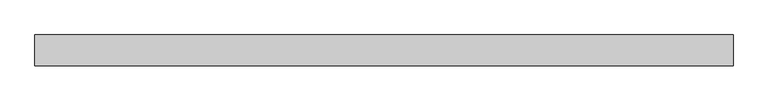
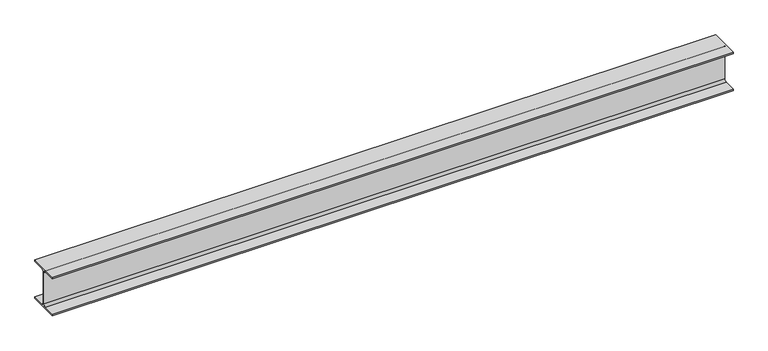
"""IFC4 building model written with IfcOpenShell, lengths in millimetres: beam geometry, 0912_Steel Framing_H-KSD3502 : H_SB_ASB_H-340x250x9x14."""

from ifc_helpers import new_model, si_unit, point, frame, frame_2d, origin, place, context, project, spatial, polyline, circle_curve, trimmed, segment, composite_curve, outline, extrude, source, transform, mapped, element, save


def beam_b7f7b6e9(model_context):
    return source(origin(), model_context, "Body", "SweptSolid", [
        extrude(outline(composite_curve([segment(polyline([(125.0, -156.0), (125.0, -170.0), (-125.0, -170.0), (-125.0, -156.0), (-24.5, -156.0)]), True, "CONTINUOUS"), segment(trimmed(circle_curve(frame_2d((-24.5, -136.0)), 20.0), [point((-24.5, -156.0))], [point((-4.5, -136.0))], True, "CARTESIAN"), True, "CONTINUOUS"), segment(polyline([(-4.5, -136.0), (-4.5, 136.0)]), True, "CONTINUOUS"), segment(trimmed(circle_curve(frame_2d((-24.5, 136.0)), 20.0), [point((-4.5, 136.0))], [point((-24.5, 156.0))], True, "CARTESIAN"), True, "CONTINUOUS"), segment(polyline([(-24.5, 156.0), (-125.0, 156.0), (-125.0, 170.0), (125.0, 170.0), (125.0, 156.0), (24.5, 156.0)]), True, "CONTINUOUS"), segment(trimmed(circle_curve(frame_2d((24.5, 136.0)), 20.0), [point((24.5, 156.0))], [point((4.5, 136.0))], True, "CARTESIAN"), True, "CONTINUOUS"), segment(polyline([(4.5, 136.0), (4.5, -136.0)]), True, "CONTINUOUS"), segment(trimmed(circle_curve(frame_2d((24.5, -136.0)), 20.0), [point((4.5, -136.0))], [point((24.5, -156.0))], True, "CARTESIAN"), True, "CONTINUOUS"), segment(polyline([(24.5, -156.0), (125.0, -156.0)]), True, "CONTINUOUS")], self_intersect=False)), frame((-2837.3, 0.0, 0.0), z_axis=(1.0, 0.0, 0.0), x_axis=(0.0, 1.0, 0.0)), (0.0, 0.0, 1.0), 5674.6),
    ])


if __name__ == "__main__":
    model = new_model("IFC4")
    model_context = context("Model", 3, world=origin())
    ifc_project = project(units=[si_unit("LENGTHUNIT", "METRE", prefix="MILLI")], contexts=[model_context])
    site = spatial("IfcSite", under=ifc_project)
    building = spatial("IfcBuilding", under=site)
    placement = place(None, origin())
    beam_shape = beam_b7f7b6e9(model_context)
    element("IfcBeam", 1, ObjectType="0912_Steel Framing_H-KSD3502 : H_SB_ASB_H-340x250x9x14", at=placement, inside=building, context=model_context, shape_type="MappedRepresentation", body=[
        mapped(beam_shape, transform((0.0, 0.0, 0.0), x_axis=(1.0, 0.0, 0.0), y_axis=(0.0, 1.0, 0.0), z_axis=(0.0, 0.0, 1.0))),
    ])
    save(model, "model.ifc")

# Revit data of these elements
# Type "0912_Steel Framing_H-KSD3502 : H_SB_ASB_H-340x250x9x14"
#   H_WM Code_1 = "S01AA002-00001 | Main Steel Structure Fabrication Work | Shelter/Building | Medium Steel - Standard (90KG/M>Weight≥30KG/M) | Material: (   )"
#   H_WM Code_2 = "S03AA028-00001 | Main Steel Structure Erection Work | Shelter/Building | Medium Steel (90KG/M>Weight≥30KG/M) | Material: (   )"
#   H_WM Code_3 = "S01AA010-00001 | Main Steel Structure Fabrication Work | Shelter/Building | Steel Painting/Coating | for Non-Fireproofed Steel Surface, Surface Preparation, Primer, Second & Final Coat | Material: (   )"
#   H_Q'ty Cal Type Tag = "SB-Q2"
#   Width = 25.0 cm
#   Web Thickness = 0.9 cm
#   Web Fillet = 2.0 cm
#   Warping Constant = 969000.0 cm⁶
#   W = 0
#   Torsional Moment of Inertia = 53.6551 cm⁴
#   Section Area = 101.5 cm²
#   Plastic Modulus weak axis = 447.0 cm³
#   Plastic Modulus strong axis = 1410.0 cm³
#   Perimeter = 1.63 m²/m
#   Nominal Weight = 79.70 kgf/m
#   Moment of Inertia weak axis = 3650.00 cm⁴
#   Moment of Inertia strong axis = 21700.00 cm⁴
#   Height = 34.0 cm
#   Flange Thickness = 1.4 cm
#   Elastic Modulus weak axis = 292.0 cm³
#   Elastic Modulus strong axis = 1280.0 cm³
#   Centroid Vertical = 17.0 cm
#   Centroid Horizontal = 12.5 cm
#   Ix = 217000000
#   Length [instance default] = 1.5240 m
#   Zx = 1410000
#   b = 0.2500 m
#   h = 0.3400 m
#   r = 0.0200 m
#   s = 0.0090 m
#   t = 0.0140 m
#   A = 0.01015 m²
#   Structural Material [instance default] = Steel, 45-345
#   Assembly Code = ""
# Element 1 (IfcBeam, "0912_Steel Framing_H-KSD3502 : H_SB_ASB_H-340x250x9x14")
#   Structural Material = none
# Materials
#   "Steel, 45-345": class "Metal", colour RGB 189 187 185, transparency 0, Description = "Steel 345 MPa", Cost = 0
